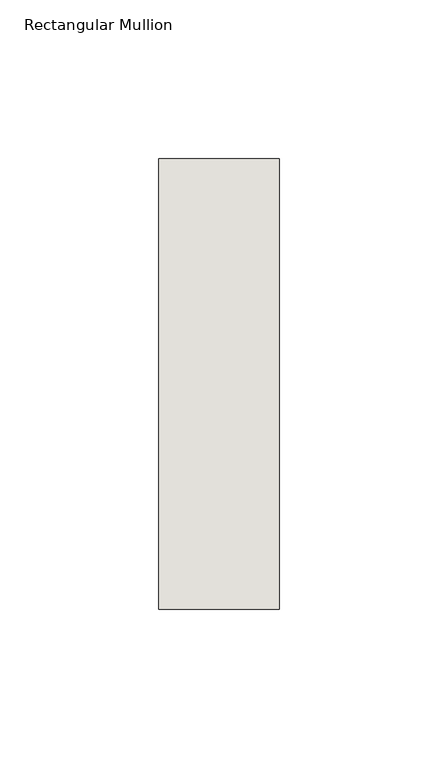
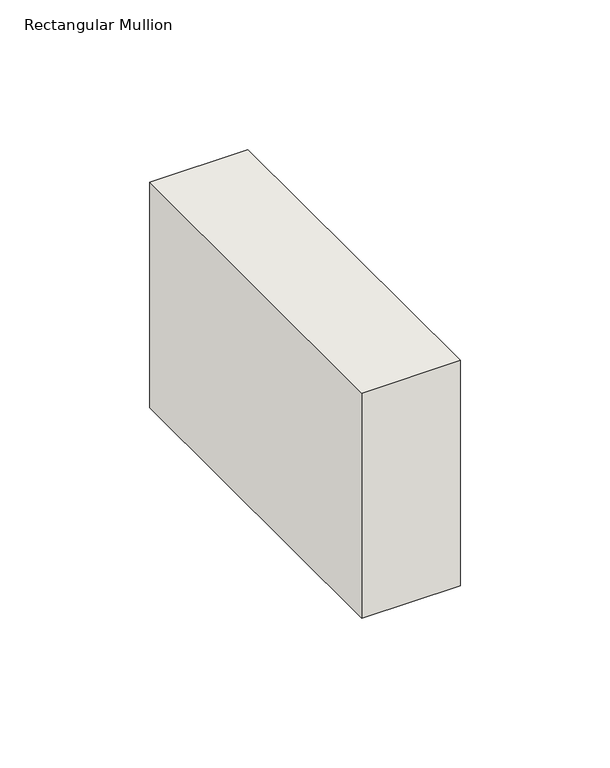
"""IFC4 building model written with IfcOpenShell, lengths in millimetres: wall geometry, Rectangular Mullion : NLRS_21_CWM_hsb-regel 38x142_gen_rsf."""

from ifc_helpers import new_model, si_unit, frame, origin, place, context, project, spatial, polyline, outline, extrude, source, transform, mapped, element, save


def rectangular_mullion_0457e6f6(model_context):
    return source(origin(), model_context, "Body", "SweptSolid", [
        extrude(outline(polyline([(19.0, -71.0), (-19.0, -71.0), (-19.0, 71.0), (19.0, 71.0), (19.0, -71.0)])), frame((0.0, 0.0, -92.0), z_axis=(0.0, 0.0, 1.0), x_axis=(1.0, 0.0, 0.0)), (0.0, 0.0, 1.0), 92.0),
    ])


if __name__ == "__main__":
    model = new_model("IFC4")
    model_context = context("Model", 3, world=origin())
    ifc_project = project(units=[si_unit("LENGTHUNIT", "METRE", prefix="MILLI")], contexts=[model_context])
    site = spatial("IfcSite", under=ifc_project)
    building = spatial("IfcBuilding", under=site)
    placement = place(None, origin())
    rectangular_mullion_shape = rectangular_mullion_0457e6f6(model_context)
    element("IfcWall", 1, ObjectType="Rectangular Mullion : NLRS_21_CWM_hsb-regel 38x142_gen_rsf", at=placement, inside=building, context=model_context, shape_type="MappedRepresentation", body=[
        mapped(rectangular_mullion_shape, transform((0.0, 0.0, 0.0), x_axis=(1.0, 0.0, 0.0), y_axis=(0.0, 1.0, 0.0), z_axis=(0.0, 0.0, 1.0))),
    ])
    save(model, "model.ifc")

# Revit data of these elements
# Type "Rectangular Mullion : NLRS_21_CWM_hsb-regel 38x142_gen_rsf"
#   Type IfcGUID = "07M7mRoiH1CR8m_RSKIwpF"
#   Assembly Code = "21.10"
#   IfcExportAs = "IfcWall"
#   built-in parameter 1007322 = 0.465879 (stored number, unit not read)
#   built-in parameter 1007321 = 0.062336 (stored number, unit not read)
#   built-in parameter 1007320 = 0.062336 (stored number, unit not read)
# Element 1 (IfcWall, "Rectangular Mullion : NLRS_21_CWM_hsb-regel 38x142_gen_rsf")
#   Materials on its faces: "NLRS_i2_hout naaldhout vuren_gen_rsf"
# Materials
#   "NLRS_i2_hout naaldhout vuren_gen_rsf": class "I - Hout", colour RGB 234 199 147, transparency 0, Keynote = "i2", Manufacturer = "Revit Standards Foundation", URL = "www.revitstandards.org", Description = "hout vuren", Cost = 0
